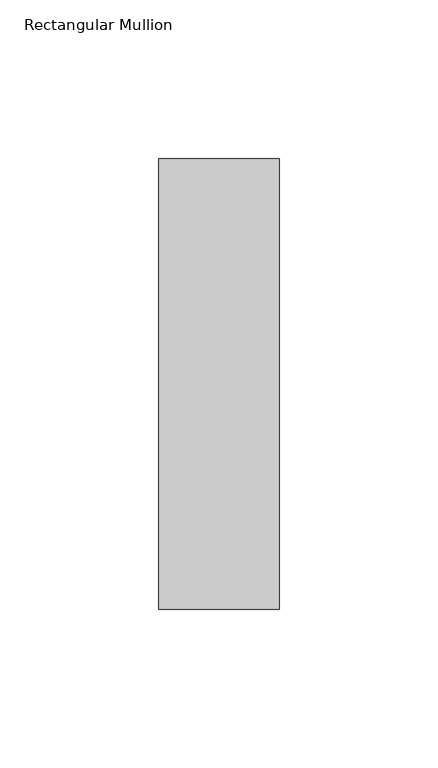
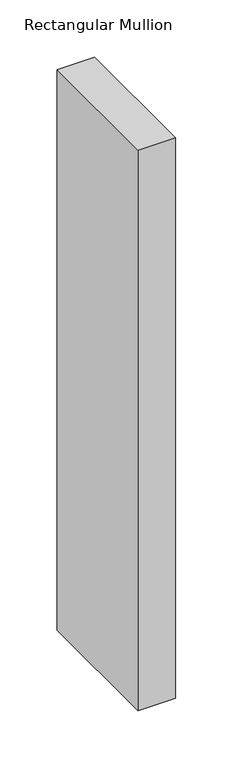
"""IFC4 building model written with IfcOpenShell, lengths in millimetres: member geometry, Rectangular Mullion : NLRS_21_CWM_hsb-regel 38x142_gen_rsf."""

from ifc_helpers import new_model, si_unit, frame, origin, place, context, project, spatial, polyline, outline, extrude, source, transform, mapped, element, save


def rectangular_mullion_45531403(model_context):
    return source(origin(), model_context, "Body", "SweptSolid", [
        extrude(outline(polyline([(19.0, -71.0), (-19.0, -71.0), (-19.0, 71.0), (19.0, 71.0), (19.0, -71.0)])), frame((0.0, 0.0, -599.0), z_axis=(0.0, 0.0, 1.0), x_axis=(1.0, 0.0, 0.0)), (0.0, 0.0, 1.0), 599.0),
    ])


if __name__ == "__main__":
    model = new_model("IFC4")
    model_context = context("Model", 3, world=origin())
    ifc_project = project(units=[si_unit("LENGTHUNIT", "METRE", prefix="MILLI")], contexts=[model_context])
    site = spatial("IfcSite", under=ifc_project)
    building = spatial("IfcBuilding", under=site)
    placement = place(None, origin())
    rectangular_mullion_shape = rectangular_mullion_45531403(model_context)
    element("IfcMember", 1, ObjectType="Rectangular Mullion : NLRS_21_CWM_hsb-regel 38x142_gen_rsf", at=placement, inside=building, context=model_context, shape_type="MappedRepresentation", body=[
        mapped(rectangular_mullion_shape, transform((0.0, 0.0, 0.0), x_axis=(1.0, 0.0, 0.0), y_axis=(0.0, 1.0, 0.0), z_axis=(0.0, 0.0, 1.0))),
    ])
    save(model, "model.ifc")

# Revit data of these elements
# Type "Rectangular Mullion : NLRS_21_CWM_hsb-regel 38x142_gen_rsf"
#   Export Type to IFC As = "IfcWall"
#   Type IfcGUID = "07M7mRoiH1CR8m_RSKIwpF"
#   Assembly Code = "21.10"
#   built-in parameter 1007322 = 0.465879 (stored number, unit not read)
#   built-in parameter 1007321 = 0.062336 (stored number, unit not read)
#   built-in parameter 1007320 = 0.062336 (stored number, unit not read)
# Element 1 (IfcMember, "Rectangular Mullion : NLRS_21_CWM_hsb-regel 38x142_gen_rsf")
#   Materials on its faces: "NLRS_i2_hout naaldhout vuren_gen_rsf"
# Materials
#   "NLRS_i2_hout naaldhout vuren_gen_rsf": class "I - Hout", colour RGB 234 199 147, transparency 0, Keynote = "i2", Manufacturer = "Revit Standards Foundation", URL = "www.revitstandards.org", Description = "hout vuren", Cost = 0
